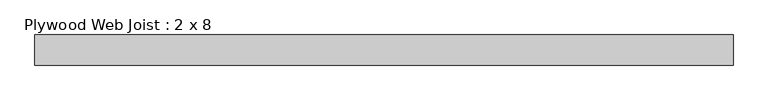
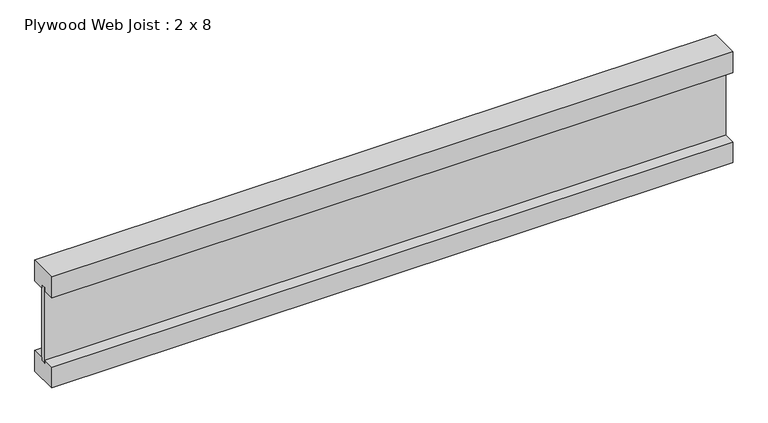
"""IFC4 building model written with IfcOpenShell, lengths in millimetres: beam geometry, Plywood Web Joist : 2 x 8."""

import ifcopenshell
import ifcopenshell.guid

model = None  # the IFC model being written
_history = None  # IfcOwnerHistory: only IFC2X3 demands one
_inside = {}  # id of a spatial element -> (the spatial element, [elements in it])
_under = {}  # id of a project, library or spatial element -> (it, [spatial elements below it])
_declared = {}  # id of a project -> (the project, [libraries it declares])
_typed = {}  # id of a type object -> (the type object, [elements of that type])
_made_of = {}  # id of a material, layer set ... -> (it, [elements and type objects made of it])


def new_model(schema):
    """Start an empty IFC model of exactly this schema.

    Asked for "IFC4X3", IfcOpenShell would pick the latest addendum, in which some entities
    have other attributes; the version numbers below select the first issue.
    IFC2X3 requires an IfcOwnerHistory on every rooted entity: one is made here for all.
    """
    global model, _history
    if schema == "IFC4X3":
        model = ifcopenshell.file(schema_version=(4, 3, 0, 0))
    else:
        model = ifcopenshell.file(schema=schema)
    _inside.clear()
    _under.clear()
    _declared.clear()
    _typed.clear()
    _made_of.clear()
    _history = None
    if model.schema == "IFC2X3":
        org = make("IfcOrganization", Name="unknown")
        user = make(
            "IfcPersonAndOrganization",
            ThePerson=make("IfcPerson", FamilyName="unknown"),
            TheOrganization=org,
        )
        app = make(
            "IfcApplication",
            ApplicationDeveloper=org,
            Version="unknown",
            ApplicationFullName="unknown",
            ApplicationIdentifier="unknown",
        )
        _history = make(
            "IfcOwnerHistory",
            OwningUser=user,
            OwningApplication=app,
            ChangeAction="ADDED",
            CreationDate=0,
        )
    return model


def make(cls, **values):
    """One entity of the class cls with the attributes given. An attribute that is None is left unset."""
    return model.create_entity(
        cls, **{name: value for name, value in values.items() if value is not None}
    )


def rooted(cls, **values):
    """An entity with a GlobalId (a new one), such as an element, a storey or a relation."""
    return make(cls, GlobalId=ifcopenshell.guid.new(), OwnerHistory=_history, **values)


def si_unit(unit_type, name, prefix=None):
    """IfcSIUnit, for example si_unit("LENGTHUNIT", "METRE", prefix="MILLI")."""
    return make("IfcSIUnit", UnitType=unit_type, Prefix=prefix, Name=name)


def assignment(units):
    """IfcUnitAssignment: the units of a project."""
    return None if units is None else make("IfcUnitAssignment", Units=units)


def point(xyz):
    """IfcCartesianPoint."""
    return None if xyz is None else make("IfcCartesianPoint", Coordinates=xyz)


def direction(xyz):
    """IfcDirection."""
    return None if xyz is None else make("IfcDirection", DirectionRatios=xyz)


def frame(location, z_axis=None, x_axis=None):
    """IfcAxis2Placement3D, a coordinate frame: its origin and axes. An axis left out is left unset."""
    return make(
        "IfcAxis2Placement3D",
        Location=point(location),
        Axis=direction(z_axis),
        RefDirection=direction(x_axis),
    )


def origin():
    """The frame at (0, 0, 0) with its axes left unset."""
    return frame((0.0, 0.0, 0.0))


def place(relative_to, where):
    """IfcLocalPlacement: puts the frame where relative to a parent placement (None: the world)."""
    return make(
        "IfcLocalPlacement", PlacementRelTo=relative_to, RelativePlacement=where
    )


def context(
    kind, dimensions, precision=None, world=None, true_north=None, identifier=None
):
    """IfcGeometricRepresentationContext, for example the 3D "Model" context."""
    return make(
        "IfcGeometricRepresentationContext",
        ContextIdentifier=identifier,
        ContextType=kind,
        CoordinateSpaceDimension=dimensions,
        Precision=precision,
        WorldCoordinateSystem=world,
        TrueNorth=true_north,
    )


def project(units=None, contexts=None):
    """IfcProject with its units and contexts."""
    return rooted(
        "IfcProject",
        Name="project",
        RepresentationContexts=contexts,
        UnitsInContext=assignment(units),
    )


def spatial(cls, under=None, at=None, **own):
    """A site, building, storey or space (cls), placed at a placement, below another one or the project."""
    s = rooted(cls, ObjectPlacement=at, **own)
    if under is not None:
        _under.setdefault(under.id(), (under, []))[1].append(s)
    return s


def polyline(points):
    """IfcPolyline through the points."""
    return make("IfcPolyline", Points=[point(p) for p in points])


def outline(outer, holes=None, kind="AREA"):
    """IfcArbitraryClosedProfileDef: a profile drawn as a closed curve; with holes, ...WithVoids."""
    if holes is None:
        return make("IfcArbitraryClosedProfileDef", ProfileType=kind, OuterCurve=outer)
    return make(
        "IfcArbitraryProfileDefWithVoids",
        ProfileType=kind,
        OuterCurve=outer,
        InnerCurves=holes,
    )


def extrude(swept, where, along, depth):
    """IfcExtrudedAreaSolid: the profile swept, set in the frame where, extruded along a direction by depth."""
    return make(
        "IfcExtrudedAreaSolid",
        SweptArea=swept,
        Position=where,
        ExtrudedDirection=direction(along),
        Depth=depth,
    )


def shape(context_of_items, identifier, shape_type, items):
    """IfcShapeRepresentation: the items that make up one representation, for example the "Body"."""
    return make(
        "IfcShapeRepresentation",
        ContextOfItems=context_of_items,
        RepresentationIdentifier=identifier,
        RepresentationType=shape_type,
        Items=items,
    )


def source(mapping_origin, context_of_items, identifier, shape_type, items):
    """IfcRepresentationMap: a shape defined once, which mapped items show again and again."""
    return make(
        "IfcRepresentationMap",
        MappingOrigin=mapping_origin,
        MappedRepresentation=shape(context_of_items, identifier, shape_type, items),
    )


def transform(
    local_origin,
    x_axis=None,
    y_axis=None,
    z_axis=None,
    scale=None,
    scale2=None,
    scale3=None,
    uniform=True,
):
    """IfcCartesianTransformationOperator3D, or its non-uniform kind. x_axis, y_axis, z_axis: its Axis1, 2, 3."""
    if uniform:
        return make(
            "IfcCartesianTransformationOperator3D",
            Axis1=direction(x_axis),
            Axis2=direction(y_axis),
            LocalOrigin=point(local_origin),
            Scale=scale,
            Axis3=direction(z_axis),
        )
    return make(
        "IfcCartesianTransformationOperator3DnonUniform",
        Axis1=direction(x_axis),
        Axis2=direction(y_axis),
        LocalOrigin=point(local_origin),
        Scale=scale,
        Axis3=direction(z_axis),
        Scale2=scale2,
        Scale3=scale3,
    )


def mapped(mapping_source, mapping_target):
    """IfcMappedItem: shows the shape of a source again, moved by a transform."""
    return make(
        "IfcMappedItem", MappingSource=mapping_source, MappingTarget=mapping_target
    )


def made_of(thing, what):
    """Note that an element or type object is made of a material, layer set ...; save() writes the relation."""
    if what is not None:
        _made_of.setdefault(what.id(), (what, []))[1].append(thing)
    return thing


def element(
    cls,
    number,
    at=None,
    inside=None,
    cuts=None,
    type_object=None,
    material=None,
    context=None,
    identifier="Body",
    shape_type=None,
    held_by="IfcProductDefinitionShape",
    body=None,
    shapes=None,
    **own,
):
    """One element of the class cls, such as IfcWall. Its Tag is "e" and its number.

    at: its placement. inside: the storey or other place that contains it. cuts: it is an
    opening in that element (IfcRelVoidsElement). A single representation is given by context,
    identifier, shape_type and body (its items); several are given by shapes. held_by: the class
    of the entity that holds the representations. save() writes the other relations.
    """
    e = rooted(cls, Tag="e%d" % number, ObjectPlacement=at, **own)
    if body is not None:
        shapes = [shape(context, identifier, shape_type, body)]
    if shapes is not None:
        e.Representation = make(held_by, Representations=shapes)
    if inside is not None:
        _inside.setdefault(inside.id(), (inside, []))[1].append(e)
    if cuts is not None:
        rooted(
            "IfcRelVoidsElement", RelatingBuildingElement=cuts, RelatedOpeningElement=e
        )
    if type_object is not None:
        _typed.setdefault(type_object.id(), (type_object, []))[1].append(e)
    return made_of(e, material)


def aggregate(whole, parts):
    """IfcRelAggregates: a whole, such as a stair, and the parts it consists of."""
    return rooted("IfcRelAggregates", RelatingObject=whole, RelatedObjects=parts)


def save(model, path):
    """Write the relations noted so far, then the file.

    IfcRelAggregates (storeys below a building ...), IfcRelContainedInSpatialStructure (elements
    in a storey), IfcRelDefinesByType, IfcRelAssociatesMaterial and IfcRelDeclares: one each for
    every whole, place, type object, material and project.
    """
    for whole, parts in _under.values():
        aggregate(whole, parts)
    for where, things in _inside.values():
        rooted(
            "IfcRelContainedInSpatialStructure",
            RelatedElements=things,
            RelatingStructure=where,
        )
    for kind, things in _typed.values():
        rooted("IfcRelDefinesByType", RelatedObjects=things, RelatingType=kind)
    for what, things in _made_of.values():
        rooted("IfcRelAssociatesMaterial", RelatedObjects=things, RelatingMaterial=what)
    for by, libraries in _declared.values():
        rooted("IfcRelDeclares", RelatingContext=by, RelatedDefinitions=libraries)
    model.write(path)


def plywood_web_joist_2_x_8_69fe57bf(model_context):
    return source(origin(), model_context, "Body", "SweptSolid", [
        extrude(outline(polyline([(-25.4, 101.6), (25.4, 101.6), (25.4, 63.5), (4.7625, 63.5), (4.7625, 69.85), (-4.7625, 69.85), (-4.7625, 63.5), (-25.4, 63.5), (-25.4, 101.6)])), frame((-589.0383025, 0.0, 0.0), z_axis=(1.0, 0.0, 0.0), x_axis=(0.0, 1.0, 0.0)), (0.0, 0.0, 1.0), 1178.0766049),
        extrude(outline(polyline([(25.4, -63.5), (25.4, -101.6), (-25.4, -101.6), (-25.4, -63.5), (-4.7625, -63.5), (-4.7625, -69.1160374), (4.7625, -69.1160374), (4.7625, -63.5), (25.4, -63.5)])), frame((-589.0383025, 0.0, 0.0), z_axis=(1.0, 0.0, 0.0), x_axis=(0.0, 1.0, 0.0)), (0.0, 0.0, 1.0), 1178.0766049),
        extrude(outline(polyline([(589.0383025, 4.7625), (589.0383025, -4.7625), (-589.0383025, -4.7625), (-589.0383025, 4.7625), (589.0383025, 4.7625)])), frame((0.0, 0.0, -69.1160374), z_axis=(0.0, 0.0, 1.0), x_axis=(1.0, 0.0, 0.0)), (0.0, 0.0, 1.0), 138.9660374),
    ])


if __name__ == "__main__":
    model = new_model("IFC4")
    model_context = context("Model", 3, world=origin())
    ifc_project = project(units=[si_unit("LENGTHUNIT", "METRE", prefix="MILLI")], contexts=[model_context])
    site = spatial("IfcSite", under=ifc_project)
    building = spatial("IfcBuilding", under=site)
    placement = place(None, origin())
    plywood_web_joist_2_x_8_shape = plywood_web_joist_2_x_8_69fe57bf(model_context)
    element("IfcBeam", 1, ObjectType="Plywood Web Joist : 2 x 8", at=placement, inside=building, context=model_context, shape_type="MappedRepresentation", body=[
        mapped(plywood_web_joist_2_x_8_shape, transform((0.0, 0.0, 0.0), x_axis=(1.0, 0.0, 0.0), y_axis=(0.0, 1.0, 0.0), z_axis=(0.0, 0.0, 1.0))),
    ])
    save(model, "model.ifc")

# Revit data of these elements
# Type "Plywood Web Joist : 2 x 8"
#   Assembly Code = "B10"
#   Length [instance default] = 5' - 0"
#   b = 0' - 2"
#   d = 0' - 8"
#   Structural Material [instance default] = Softwood, Lumber
# Element 1 (IfcBeam, "Plywood Web Joist : 2 x 8")
#   Materials on its faces: "Softwood, Lumber"
# Materials
#   "Softwood, Lumber": class "Wood", colour RGB 144 113 62, transparency 0, Description = "Pinus Echinata", Cost = 0
